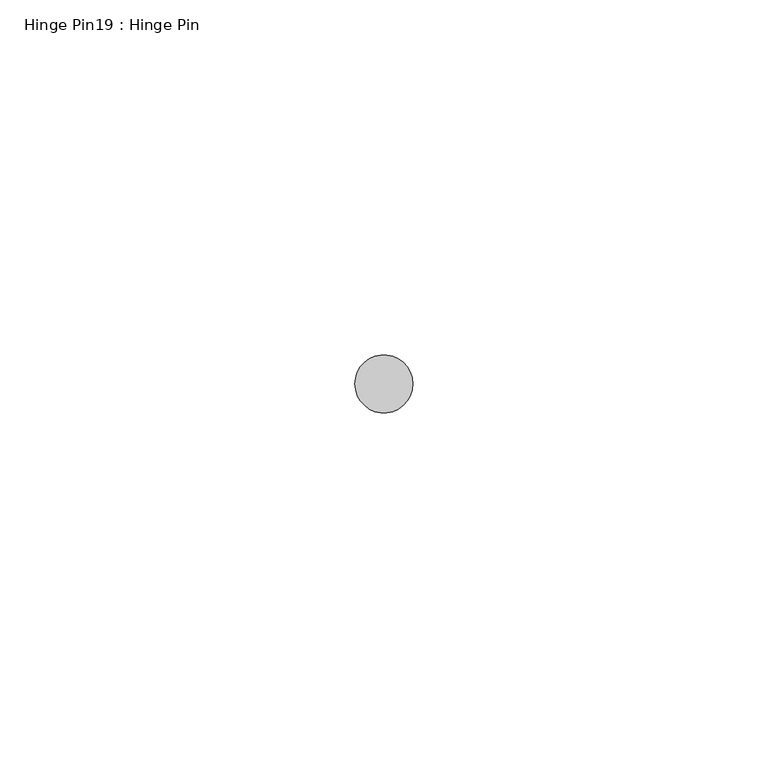
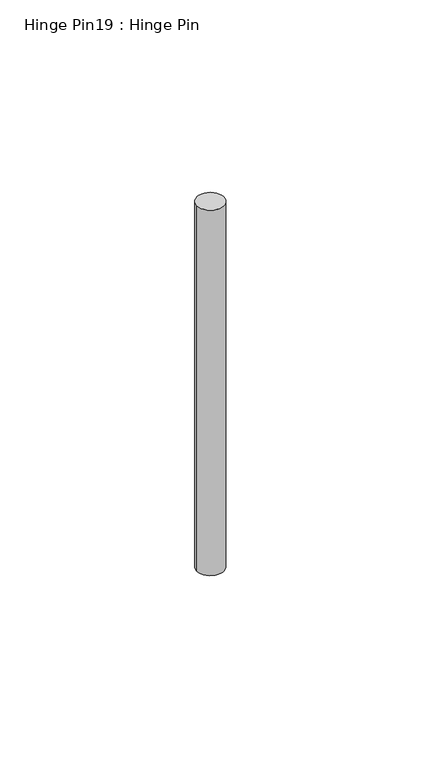
"""IFC4 building model written with IfcOpenShell, lengths in millimetres: proxy geometry, Hinge Pin19 : Hinge Pin."""

import ifcopenshell
import ifcopenshell.guid

model = None  # the IFC model being written
_history = None  # IfcOwnerHistory: only IFC2X3 demands one
_inside = {}  # id of a spatial element -> (the spatial element, [elements in it])
_under = {}  # id of a project, library or spatial element -> (it, [spatial elements below it])
_declared = {}  # id of a project -> (the project, [libraries it declares])
_typed = {}  # id of a type object -> (the type object, [elements of that type])
_made_of = {}  # id of a material, layer set ... -> (it, [elements and type objects made of it])


def new_model(schema):
    """Start an empty IFC model of exactly this schema.

    Asked for "IFC4X3", IfcOpenShell would pick the latest addendum, in which some entities
    have other attributes; the version numbers below select the first issue.
    IFC2X3 requires an IfcOwnerHistory on every rooted entity: one is made here for all.
    """
    global model, _history
    if schema == "IFC4X3":
        model = ifcopenshell.file(schema_version=(4, 3, 0, 0))
    else:
        model = ifcopenshell.file(schema=schema)
    _inside.clear()
    _under.clear()
    _declared.clear()
    _typed.clear()
    _made_of.clear()
    _history = None
    if model.schema == "IFC2X3":
        org = make("IfcOrganization", Name="unknown")
        user = make(
            "IfcPersonAndOrganization",
            ThePerson=make("IfcPerson", FamilyName="unknown"),
            TheOrganization=org,
        )
        app = make(
            "IfcApplication",
            ApplicationDeveloper=org,
            Version="unknown",
            ApplicationFullName="unknown",
            ApplicationIdentifier="unknown",
        )
        _history = make(
            "IfcOwnerHistory",
            OwningUser=user,
            OwningApplication=app,
            ChangeAction="ADDED",
            CreationDate=0,
        )
    return model


def make(cls, **values):
    """One entity of the class cls with the attributes given. An attribute that is None is left unset."""
    return model.create_entity(
        cls, **{name: value for name, value in values.items() if value is not None}
    )


def rooted(cls, **values):
    """An entity with a GlobalId (a new one), such as an element, a storey or a relation."""
    return make(cls, GlobalId=ifcopenshell.guid.new(), OwnerHistory=_history, **values)


def si_unit(unit_type, name, prefix=None):
    """IfcSIUnit, for example si_unit("LENGTHUNIT", "METRE", prefix="MILLI")."""
    return make("IfcSIUnit", UnitType=unit_type, Prefix=prefix, Name=name)


def assignment(units):
    """IfcUnitAssignment: the units of a project."""
    return None if units is None else make("IfcUnitAssignment", Units=units)


def point(xyz):
    """IfcCartesianPoint."""
    return None if xyz is None else make("IfcCartesianPoint", Coordinates=xyz)


def direction(xyz):
    """IfcDirection."""
    return None if xyz is None else make("IfcDirection", DirectionRatios=xyz)


def frame(location, z_axis=None, x_axis=None):
    """IfcAxis2Placement3D, a coordinate frame: its origin and axes. An axis left out is left unset."""
    return make(
        "IfcAxis2Placement3D",
        Location=point(location),
        Axis=direction(z_axis),
        RefDirection=direction(x_axis),
    )


def frame_2d(location, x_axis=None):
    """IfcAxis2Placement2D, a coordinate frame in the plane: its origin and x axis."""
    return make(
        "IfcAxis2Placement2D", Location=point(location), RefDirection=direction(x_axis)
    )


def origin():
    """The frame at (0, 0, 0) with its axes left unset."""
    return frame((0.0, 0.0, 0.0))


def place(relative_to, where):
    """IfcLocalPlacement: puts the frame where relative to a parent placement (None: the world)."""
    return make(
        "IfcLocalPlacement", PlacementRelTo=relative_to, RelativePlacement=where
    )


def context(
    kind, dimensions, precision=None, world=None, true_north=None, identifier=None
):
    """IfcGeometricRepresentationContext, for example the 3D "Model" context."""
    return make(
        "IfcGeometricRepresentationContext",
        ContextIdentifier=identifier,
        ContextType=kind,
        CoordinateSpaceDimension=dimensions,
        Precision=precision,
        WorldCoordinateSystem=world,
        TrueNorth=true_north,
    )


def project(units=None, contexts=None):
    """IfcProject with its units and contexts."""
    return rooted(
        "IfcProject",
        Name="project",
        RepresentationContexts=contexts,
        UnitsInContext=assignment(units),
    )


def spatial(cls, under=None, at=None, **own):
    """A site, building, storey or space (cls), placed at a placement, below another one or the project."""
    s = rooted(cls, ObjectPlacement=at, **own)
    if under is not None:
        _under.setdefault(under.id(), (under, []))[1].append(s)
    return s


def circle_curve(where, radius):
    """IfcCircle in the frame where."""
    return make("IfcCircle", Position=where, Radius=radius)


def trimmed(basis, trim1, trim2, sense, master):
    """IfcTrimmedCurve: the piece of a basis curve between two trims."""
    return make(
        "IfcTrimmedCurve",
        BasisCurve=basis,
        Trim1=trim1,
        Trim2=trim2,
        SenseAgreement=sense,
        MasterRepresentation=master,
    )


def segment(curve, same_sense, transition):
    """IfcCompositeCurveSegment."""
    return make(
        "IfcCompositeCurveSegment",
        Transition=transition,
        SameSense=same_sense,
        ParentCurve=curve,
    )


def composite_curve(segments, self_intersect=None):
    """IfcCompositeCurve: segments joined end to end."""
    return make("IfcCompositeCurve", Segments=segments, SelfIntersect=self_intersect)


def outline(outer, holes=None, kind="AREA"):
    """IfcArbitraryClosedProfileDef: a profile drawn as a closed curve; with holes, ...WithVoids."""
    if holes is None:
        return make("IfcArbitraryClosedProfileDef", ProfileType=kind, OuterCurve=outer)
    return make(
        "IfcArbitraryProfileDefWithVoids",
        ProfileType=kind,
        OuterCurve=outer,
        InnerCurves=holes,
    )


def extrude(swept, where, along, depth):
    """IfcExtrudedAreaSolid: the profile swept, set in the frame where, extruded along a direction by depth."""
    return make(
        "IfcExtrudedAreaSolid",
        SweptArea=swept,
        Position=where,
        ExtrudedDirection=direction(along),
        Depth=depth,
    )


def shape(context_of_items, identifier, shape_type, items):
    """IfcShapeRepresentation: the items that make up one representation, for example the "Body"."""
    return make(
        "IfcShapeRepresentation",
        ContextOfItems=context_of_items,
        RepresentationIdentifier=identifier,
        RepresentationType=shape_type,
        Items=items,
    )


def source(mapping_origin, context_of_items, identifier, shape_type, items):
    """IfcRepresentationMap: a shape defined once, which mapped items show again and again."""
    return make(
        "IfcRepresentationMap",
        MappingOrigin=mapping_origin,
        MappedRepresentation=shape(context_of_items, identifier, shape_type, items),
    )


def transform(
    local_origin,
    x_axis=None,
    y_axis=None,
    z_axis=None,
    scale=None,
    scale2=None,
    scale3=None,
    uniform=True,
):
    """IfcCartesianTransformationOperator3D, or its non-uniform kind. x_axis, y_axis, z_axis: its Axis1, 2, 3."""
    if uniform:
        return make(
            "IfcCartesianTransformationOperator3D",
            Axis1=direction(x_axis),
            Axis2=direction(y_axis),
            LocalOrigin=point(local_origin),
            Scale=scale,
            Axis3=direction(z_axis),
        )
    return make(
        "IfcCartesianTransformationOperator3DnonUniform",
        Axis1=direction(x_axis),
        Axis2=direction(y_axis),
        LocalOrigin=point(local_origin),
        Scale=scale,
        Axis3=direction(z_axis),
        Scale2=scale2,
        Scale3=scale3,
    )


def mapped(mapping_source, mapping_target):
    """IfcMappedItem: shows the shape of a source again, moved by a transform."""
    return make(
        "IfcMappedItem", MappingSource=mapping_source, MappingTarget=mapping_target
    )


def made_of(thing, what):
    """Note that an element or type object is made of a material, layer set ...; save() writes the relation."""
    if what is not None:
        _made_of.setdefault(what.id(), (what, []))[1].append(thing)
    return thing


def element(
    cls,
    number,
    at=None,
    inside=None,
    cuts=None,
    type_object=None,
    material=None,
    context=None,
    identifier="Body",
    shape_type=None,
    held_by="IfcProductDefinitionShape",
    body=None,
    shapes=None,
    **own,
):
    """One element of the class cls, such as IfcWall. Its Tag is "e" and its number.

    at: its placement. inside: the storey or other place that contains it. cuts: it is an
    opening in that element (IfcRelVoidsElement). A single representation is given by context,
    identifier, shape_type and body (its items); several are given by shapes. held_by: the class
    of the entity that holds the representations. save() writes the other relations.
    """
    e = rooted(cls, Tag="e%d" % number, ObjectPlacement=at, **own)
    if body is not None:
        shapes = [shape(context, identifier, shape_type, body)]
    if shapes is not None:
        e.Representation = make(held_by, Representations=shapes)
    if inside is not None:
        _inside.setdefault(inside.id(), (inside, []))[1].append(e)
    if cuts is not None:
        rooted(
            "IfcRelVoidsElement", RelatingBuildingElement=cuts, RelatedOpeningElement=e
        )
    if type_object is not None:
        _typed.setdefault(type_object.id(), (type_object, []))[1].append(e)
    return made_of(e, material)


def aggregate(whole, parts):
    """IfcRelAggregates: a whole, such as a stair, and the parts it consists of."""
    return rooted("IfcRelAggregates", RelatingObject=whole, RelatedObjects=parts)


def save(model, path):
    """Write the relations noted so far, then the file.

    IfcRelAggregates (storeys below a building ...), IfcRelContainedInSpatialStructure (elements
    in a storey), IfcRelDefinesByType, IfcRelAssociatesMaterial and IfcRelDeclares: one each for
    every whole, place, type object, material and project.
    """
    for whole, parts in _under.values():
        aggregate(whole, parts)
    for where, things in _inside.values():
        rooted(
            "IfcRelContainedInSpatialStructure",
            RelatedElements=things,
            RelatingStructure=where,
        )
    for kind, things in _typed.values():
        rooted("IfcRelDefinesByType", RelatedObjects=things, RelatingType=kind)
    for what, things in _made_of.values():
        rooted("IfcRelAssociatesMaterial", RelatedObjects=things, RelatingMaterial=what)
    for by, libraries in _declared.values():
        rooted("IfcRelDeclares", RelatingContext=by, RelatedDefinitions=libraries)
    model.write(path)


def hinge_pin19_hinge_pin_9f56c2fe(model_context):
    return source(origin(), model_context, "Body", "SweptSolid", [
        extrude(outline(composite_curve([segment(trimmed(circle_curve(frame_2d((587319.1320739, -534100.7049841)), 4.0894), [point((587315.0426739, -534100.7049841))], [point((587323.2214739, -534100.7049841))], False, "CARTESIAN"), True, "CONTINUOUS"), segment(trimmed(circle_curve(frame_2d((587319.1320739, -534100.7049841)), 4.0894), [point((587323.2214739, -534100.7049841))], [point((587315.0426739, -534100.7049841))], False, "CARTESIAN"), True, "CONTINUOUS")], self_intersect=False)), frame((0.0, 0.0, 1941.3140625), z_axis=(0.0, 0.0, 1.0), x_axis=(1.0, 0.0, 0.0)), (0.0, 0.0, 1.0), 117.871875),
    ])


if __name__ == "__main__":
    model = new_model("IFC4")
    model_context = context("Model", 3, world=origin())
    ifc_project = project(units=[si_unit("LENGTHUNIT", "METRE", prefix="MILLI")], contexts=[model_context])
    site = spatial("IfcSite", under=ifc_project)
    building = spatial("IfcBuilding", under=site)
    placement = place(None, origin())
    hinge_pin19_hinge_pin_shape = hinge_pin19_hinge_pin_9f56c2fe(model_context)
    element("IfcBuildingElementProxy", 1, Name="Hinge Pin19 : Hinge Pin", ObjectType="Hinge Pin19 : Hinge Pin", at=placement, inside=building, context=model_context, shape_type="MappedRepresentation", body=[
        mapped(hinge_pin19_hinge_pin_shape, transform((0.0, 0.0, 0.0), x_axis=(1.0, 0.0, 0.0), y_axis=(0.0, 1.0, 0.0), z_axis=(0.0, 0.0, 1.0))),
    ])
    save(model, "model.ifc")

# Revit data of these elements
# Element 1 (IfcBuildingElementProxy, "Hinge Pin19 : Hinge Pin")
#   Materials on its faces: "6\"X6\" WELD-ON STL BUTT HINGE"
# Materials
#   "6\"X6\" WELD-ON STL BUTT HINGE": class "Metal", colour RGB 189 187 185, transparency 0, Description = "Carbon steel", Cost = 0
